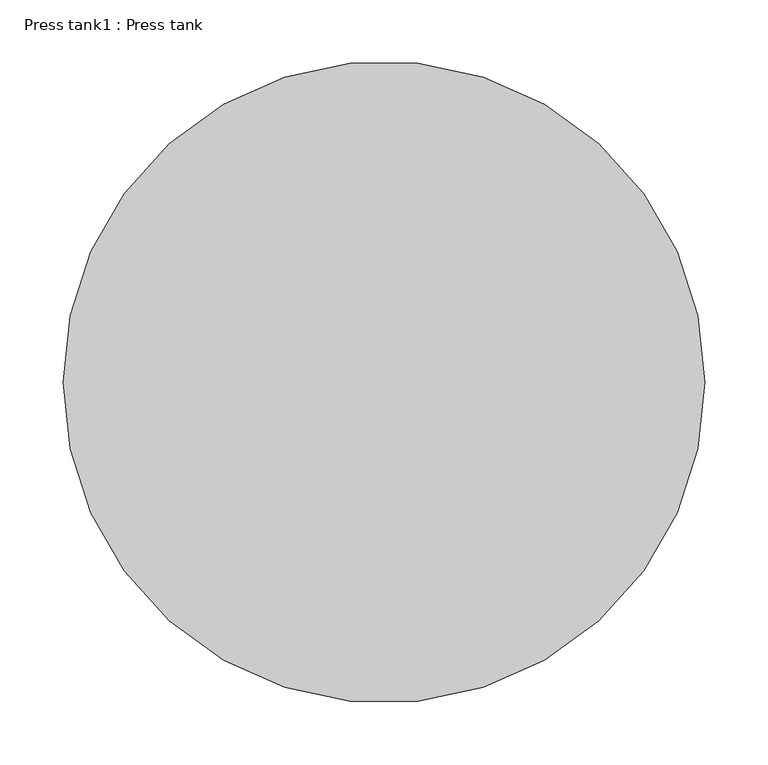
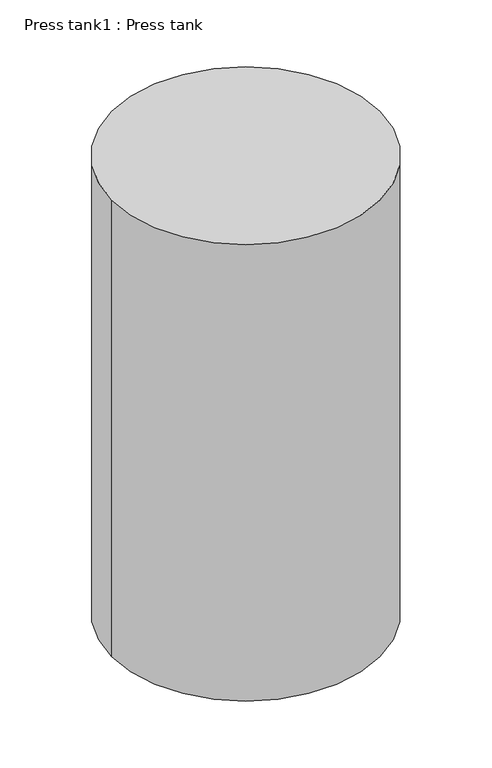
"""IFC4 building model written with IfcOpenShell, lengths in millimetres: proxy geometry, Press tank1 : Press tank."""

from ifc_helpers import new_model, si_unit, point, frame, frame_2d, origin, place, context, project, spatial, circle_curve, trimmed, segment, composite_curve, outline, extrude, source, transform, mapped, element, save


def press_tank1_press_tank_732dd890(model_context):
    return source(origin(), model_context, "Body", "SweptSolid", [
        extrude(outline(composite_curve([segment(trimmed(circle_curve(frame_2d((26385.9004782, 10738.3240491)), 254.0), [point((26131.9004782, 10738.3240491))], [point((26639.9004782, 10738.3240491))], False, "CARTESIAN"), True, "CONTINUOUS"), segment(trimmed(circle_curve(frame_2d((26385.9004782, 10738.3240491)), 254.0), [point((26639.9004782, 10738.3240491))], [point((26131.9004782, 10738.3240491))], False, "CARTESIAN"), True, "CONTINUOUS")], self_intersect=False)), frame((0.0, 0.0, 2832.1), z_axis=(0.0, 0.0, 1.0), x_axis=(1.0, 0.0, 0.0)), (0.0, 0.0, 1.0), 914.4),
    ])


if __name__ == "__main__":
    model = new_model("IFC4")
    model_context = context("Model", 3, world=origin())
    ifc_project = project(units=[si_unit("LENGTHUNIT", "METRE", prefix="MILLI")], contexts=[model_context])
    site = spatial("IfcSite", under=ifc_project)
    building = spatial("IfcBuilding", under=site)
    placement = place(None, origin())
    press_tank1_press_tank_shape = press_tank1_press_tank_732dd890(model_context)
    element("IfcBuildingElementProxy", 1, Name="Press tank1 : Press tank", ObjectType="Press tank1 : Press tank", at=placement, inside=building, context=model_context, shape_type="MappedRepresentation", body=[
        mapped(press_tank1_press_tank_shape, transform((0.0, 0.0, 0.0), x_axis=(1.0, 0.0, 0.0), y_axis=(0.0, 1.0, 0.0), z_axis=(0.0, 0.0, 1.0))),
    ])
    save(model, "model.ifc")
